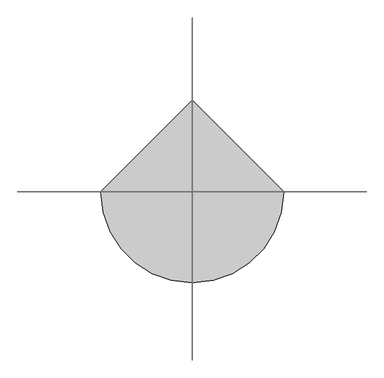
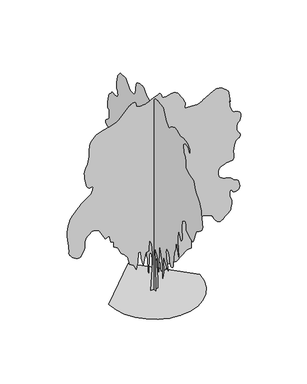
"""IFC4 building model written with IfcOpenShell, lengths in millimetres: proxy geometry, goldenchain 26164 : goldenchain 26164."""

from ifc_helpers import new_model, si_unit, origin, place, context, project, spatial, triangles, source, transform, mapped, element, save


def entourage_92130817(model_context):
    return source(origin(), model_context, "Body", "Tessellation", [
        triangles([(-0.0021439, 84.0442886, 0.0017013), (-0.0021439, -79.514705, 0.0017013), (-0.0021439, -54.9808464, 768.7285137), (-0.0021439, -30.4472354, 1202.1592524), (-0.0021439, -128.5824313, 1087.6687117), (-0.0021439, -161.2943336, 981.3544888), (-0.0021439, -161.2943336, 776.9073023), (-0.0021439, -202.1840252, 613.3465736), (-0.0021439, -226.7178838, 1406.6089096), (-0.0021439, -292.140671, 1251.2269695), (-0.0021439, -390.2761053, 932.2867716), (-0.0021439, -406.6337188, 556.102575), (-0.0021439, -447.5226474, 752.37348), (-0.0021439, -422.9887888, 1120.3813951), (-0.0021439, -398.4548939, 1226.6931473), (-0.0021439, -562.0131517, 1022.2459608), (-0.0021439, -643.7935524, 907.7528767), (-0.0021439, -570.1919403, 1161.2703238), (-0.0021439, -564.9696937, 1199.7284414), (-0.0021439, -559.9633495, 1237.6125389), (-0.0021439, -555.386267, 1274.3536102), (-0.0021439, -551.4518414, 1309.3777805), (-0.0021439, -548.3758664, 1342.1157532), (-0.0021439, -546.37181, 1371.9887844), (-0.0021439, -545.6580817, 1398.4301937), (-0.0021439, -546.8493608, 1421.534016), (-0.0021439, -550.1869114, 1442.0622688), (-0.0021439, -555.312616, 1460.4442863), (-0.0021439, -561.8709002, 1477.1091122), (-0.0021439, -569.5010668, 1492.488842), (-0.0021439, -577.8449615, 1507.0100487), (-0.0021439, -586.5470103, 1521.0994503), (-0.0021439, -614.3955648, 1489.5551548), (-0.0021439, -641.0985861, 1458.0134754), (-0.0021439, -665.5130842, 1426.4691799), (-0.0021439, -686.4960331, 1394.9248844), (-0.0021439, -702.8993196, 1363.383205), (-0.0021439, -713.5800631, 1331.8389095), (-0.0021439, -717.3950918, 1300.294614), (-0.0021439, -719.0638853, 1269.9442863), (-0.0021439, -723.7375099, 1241.7375778), (-0.0021439, -730.9130167, 1215.3215303), (-0.0021439, -740.0925436, 1190.333012), (-0.0021439, -750.773287, 1166.4189194), (-0.0021439, -762.4572395, 1143.2210621), (-0.0021439, -774.6391268, 1120.3813951), (-0.0021439, -797.2654346, 1120.6430071), (-0.0021439, -818.9620754, 1122.4794502), (-0.0021439, -838.7995274, 1127.4629396), (-0.0021439, -855.847978, 1137.1656904), (-0.0021439, -869.1753622, 1153.1626064), (-0.0021439, -877.8545563, 1177.0309896), (-0.0021439, -880.9533497, 1210.3380409), (-0.0021439, -882.6221432, 1252.4664288), (-0.0021439, -887.2956951, 1301.0338131), (-0.0021439, -894.4712019, 1354.9656956), (-0.0021439, -903.6508015, 1413.1900486), (-0.0021439, -914.3314722, 1474.6301937), (-0.0021439, -926.0154974, 1538.2190449), (-0.0021439, -938.1998554, 1602.8797783), (-0.0021439, -1003.6226789, 1758.2592476), (-0.0021439, -1028.1565012, 2036.3105896), (-0.0021439, -1134.4707968, 1611.0560234), (-0.0021439, -1093.5793247, 2028.1317284), (-0.0021439, -1118.113147, 2379.7846825), (-0.0021439, -1257.140126, 2134.4460239), (-0.0021439, -1267.5820759, 2148.5354256), (-0.0021439, -1277.5946915, 2163.0564869), (-0.0021439, -1286.7514, 2178.433746), (-0.0021439, -1294.6202511, 2195.1011879), (-0.0021439, -1300.7697304, 2213.4832054), (-0.0021439, -1304.7752998, 2234.0114582), (-0.0021439, -1306.2077705, 2257.1152805), (-0.0021439, -1304.3942184, 2284.415213), (-0.0021439, -1299.7206665, 2316.2921917), (-0.0021439, -1293.332539, 2351.3162167), (-0.0021439, -1286.3704639, 2388.0574333), (-0.0021439, -1279.9797203, 2425.0855511), (-0.0021439, -1275.3061684, 2460.9680992), (-0.0021439, -1273.4950871, 2494.2750778), (-0.0021439, -1274.6864388, 2526.5329926), (-0.0021439, -1278.0264965, 2560.0917), (-0.0021439, -1283.1522011, 2594.7116798), (-0.0021439, -1289.7079056, 2630.1702713), (-0.0021439, -1297.3381084, 2666.2889969), (-0.0021439, -1305.6820759, 2702.8396729), (-0.0021439, -1314.3840157, 2739.6188232), (-0.0021439, -1345.7607342, 2756.763707), (-0.0021439, -1376.1364964, 2771.6226837), (-0.0021439, -1404.5083111, 2781.8845573), (-0.0021439, -1429.8778381, 2785.2881287), (-0.0021439, -1451.239325, 2779.5474907), (-0.0021439, -1467.5969021, 2762.351738), (-0.0021439, -1477.9423462, 2731.439962), (-0.0021439, -1480.7337456, 2695.2194984), (-0.0021439, -1478.2292473, 2663.0124527), (-0.0021439, -1475.1534176, 2633.802317), (-0.0021439, -1476.2277706, 2606.5990356), (-0.0021439, -1486.169315, 2580.3861008), (-0.0021439, -1509.7024715, 2554.1987457), (-0.0021439, -1551.5464291, 2526.9879066), (-0.0021439, -1602.9255604, 2498.8777039), (-0.0021439, -1651.1601162, 2472.3397888), (-0.0021439, -1695.0995853, 2449.9522018), (-0.0021439, -1733.6059559, 2434.2878963), (-0.0021439, -1765.5313328, 2427.9227325), (-0.0021439, -1789.7298557, 2433.4293732), (-0.0021439, -1805.0613327, 2453.3862946), (-0.0021439, -1952.2644115, 2813.2027039), (-0.0021439, -2091.2889198, 2911.3481667), (-0.0021439, -2128.6269024, 2939.9231667), (-0.0021439, -2162.6730801, 2969.615831), (-0.0021439, -2192.1420662, 3000.6293449), (-0.0021439, -2215.746294, 3033.039576), (-0.0021439, -2232.1979061, 3067.0502907), (-0.0021439, -2240.209045, 3102.7626457), (-0.0021439, -2238.4919987, 3140.329248), (-0.0021439, -2229.7188423, 3187.039769), (-0.0021439, -2218.3701164, 3246.6282829), (-0.0021439, -2205.8758209, 3313.9381279), (-0.0021439, -2193.6685719, 3383.8138046), (-0.0021439, -2183.1783691, 3451.1236496), (-0.0021439, -2175.835358, 3510.7121635), (-0.0021439, -2173.0692478, 3557.3973953), (-0.0021439, -2164.9616032, 3599.7645767), (-0.0021439, -2142.2641514, 3649.0150589), (-0.0021439, -2107.4077034, 3703.9553101), (-0.0021439, -2062.820454, 3763.492955), (-0.0021439, -2010.9410625, 3826.4594604), (-0.0021439, -1954.194817, 3891.7374527), (-0.0021439, -1895.0179058, 3958.1331093), (-0.0021439, -1837.7740162, 4187.1141907), (-0.0021439, -1625.145425, 4236.1870674), (-0.0021439, -1453.4109947, 4317.9495186), (-0.0021439, -1454.7444889, 4324.4773178), (-0.0021439, -1458.0820759, 4341.9779938), (-0.0021439, -1462.4229446, 4367.5302132), (-0.0021439, -1466.7611973, 4398.0611984), (-0.0021439, -1470.0987843, 4430.6240364), (-0.0021439, -1471.4347492, 4462.1453682), (-0.0021439, -1469.7661011, 4489.7044418), (-0.0021439, -1464.1145565, 4515.6630318), (-0.0021439, -1454.6022011, 4544.1874535), (-0.0021439, -1441.8692574, 4574.8704643), (-0.0021439, -1426.5632149, 4607.280986), (-0.0021439, -1409.3241508, 4640.9614883), (-0.0021439, -1390.7999908, 4675.5308899), (-0.0021439, -1371.6305214, 4710.506662), (-0.0021439, -1338.9179832, 4906.7725891), (-0.0021439, -1445.2321335, 4996.7391907), (-0.0021439, -1576.0802513, 4972.2028976), (-0.0021439, -1649.6793926, 4865.8782829), (-0.0021439, -1649.6793926, 4964.0237457), (-0.0021439, -1535.1888519, 5070.3230713), (-0.0021439, -1347.0966991, 5094.8593643), (-0.0021439, -1199.8935476, 5062.1439194), (-0.0021439, -1052.6903961, 5143.9319504), (-0.0021439, -946.3761005, 5152.1111023), (-0.0021439, -938.5555023, 5148.3770279), (-0.0021439, -917.8620707, 5138.3694992), (-0.0021439, -888.4387213, 5123.7901566), (-0.0021439, -854.4407965, 5106.3400589), (-0.0021439, -820.0111393, 5087.7220093), (-0.0021439, -789.3025486, 5069.7132248), (-0.0021439, -766.462809, 5053.9653488), (-0.0021439, -750.6792521, 5038.3697891), (-0.0021439, -737.326506, 5021.3516418), (-0.0021439, -724.8322105, 5005.4770294), (-0.0021439, -711.6242231, 4993.3103302), (-0.0021439, -696.1277126, 4987.4426651), (-0.0021439, -676.7678478, 4990.465155), (-0.0021439, -651.9697975, 5004.8927628), (-0.0021439, -625.6020756, 5027.117569), (-0.0021439, -602.236605, 5051.5015457), (-0.0021439, -581.3730165, 5077.6383224), (-0.0021439, -562.5135209, 5105.2226852), (-0.0021439, -545.1577126, 5133.8994232), (-0.0021439, -528.8000991, 5163.2615845), (-0.0021439, -512.9454346, 5193.0051178), (-0.0021439, -414.8099639, 5397.4496155), (-0.0021439, -169.4723773, 5438.343631), (-0.0021439, -163.4401146, 5438.1913147), (-0.0021439, -147.2511773, 5437.2006775), (-0.0021439, -123.7660828, 5434.4828201), (-0.0021439, -95.8466569, 5429.1744232), (-0.0021439, -66.3536942, 5420.4621643), (-0.0021439, -38.1480076, 5407.4315643), (-0.0021439, -14.0911332, 5389.2710449), (-0.0021439, 3.3375856, 5370.932048), (-0.0021439, 15.1871941, 5356.7590759), (-0.0021439, 23.8896415, 5344.846431), (-0.0021439, 31.8767493, 5333.3907349), (-0.0021439, 41.5805652, 5320.4874527), (-0.0021439, 55.4332171, 5304.2826279), (-0.0021439, 75.8662495, 5282.9461395), (-0.0021439, 96.8951667, 5258.2575302), (-0.0021439, 112.9172356, 5234.5595581), (-0.0021439, 126.936765, 5213.8584961), (-0.0021439, 141.9573053, 5198.1611984), (-0.0021439, 160.9836875, 5189.5000992), (-0.0021439, 187.019453, 5189.8297302), (-0.0021439, 223.0691603, 5201.1836884), (-0.0021439, 263.6977487, 5220.8435349), (-0.0021439, 301.7494776, 5244.3891907), (-0.0021439, 337.654935, 5271.1352325), (-0.0021439, 371.8458713, 5300.4468155), (-0.0021439, 404.7490228, 5331.7146744), (-0.0021439, 436.7936874, 5364.2516418), (-0.0021439, 468.4065107, 5397.4496155), (-0.0021439, 491.2487575, 5406.0857162), (-0.0021439, 514.4465784, 5413.9090759), (-0.0021439, 538.360671, 5420.1825302), (-0.0021439, 563.3491894, 5424.0945007), (-0.0021439, 589.7652005, 5424.8560822), (-0.0021439, 617.9718727, 5421.6812759), (-0.0021439, 648.3223457, 5413.807338), (-0.0021439, 679.72181, 5404.5108124), (-0.0021439, 710.2653671, 5396.4845581), (-0.0021439, 739.0892618, 5388.0513519), (-0.0021439, 765.3401304, 5377.4595566), (-0.0021439, 788.156979, 5363.0069504), (-0.0021439, 806.6837551, 5342.991893), (-0.0021439, 820.0593922, 5315.6615845), (-0.0021439, 829.6199278, 5284.3687271), (-0.0021439, 837.4634897, 5253.4822403), (-0.0021439, 843.8769791, 5222.9771255), (-0.0021439, 849.1474422, 5192.7254837), (-0.0021439, 853.5569115, 5162.7284775), (-0.0021439, 857.3973747, 5132.8326279), (-0.0021439, 860.9483208, 5103.0379349), (-0.0021439, 866.3610718, 5073.4217194), (-0.0021439, 872.7034172, 5044.897879), (-0.0021439, 880.9050968, 5018.507048), (-0.0021439, 891.895705, 4995.3166031), (-0.0021439, 906.6073797, 4976.4444992), (-0.0021439, 925.9672445, 4962.9063721), (-0.0021439, 950.90751, 4955.8451752), (-0.0021439, 981.1385862, 4952.5180527), (-0.0021439, 1014.5192522, 4950.3588821), (-0.0021439, 1049.1851595, 4950.4606201), (-0.0021439, 1083.27959, 4954.016217), (-0.0021439, 1114.9432823, 4962.1442093), (-0.0021439, 1142.314286, 4976.0125488), (-0.0021439, 1163.533485, 4996.7391907), (-0.0021439, 1185.0142233, 5025.1618744), (-0.0021439, 1212.2201935, 5059.0452713), (-0.0021439, 1241.8544312, 5094.7832062), (-0.0021439, 1270.6326164, 5128.8195007), (-0.0021439, 1295.2629444, 5157.546817), (-0.0021439, 1312.4536102, 5177.4095581), (-0.0021439, 1318.9129543, 5184.8259659), (-0.0021439, 1572.4303288, 5168.4688248), (-0.0021439, 1670.5657631, 5045.7867783), (-0.0021439, 1675.8337555, 5036.8204651), (-0.0021439, 1681.1752899, 5026.6606201), (-0.0021439, 1686.6592575, 5014.0363907), (-0.0021439, 1692.3589096, 4997.7804062), (-0.0021439, 1698.3406666, 4976.6479752), (-0.0021439, 1704.683012, 4949.4444031), (-0.0021439, 1711.4546917, 4914.9511597), (-0.0021439, 1717.9875778, 4876.8767395), (-0.0021439, 1723.6619408, 4839.6656387), (-0.0021439, 1728.6225391, 4803.1402519), (-0.0021439, 1733.00919, 4767.2247116), (-0.0021439, 1736.9665066, 4731.7155418), (-0.0021439, 1740.6392475, 4696.5112953), (-0.0021439, 1744.1673752, 4661.4337852), (-0.0021439, 1726.808987, 4636.8466232), (-0.0021439, 1710.4538807, 4611.9798271), (-0.0021439, 1696.1003963, 4586.5546349), (-0.0021439, 1684.7516705, 4560.2402527), (-0.0021439, 1677.408514, 4532.8082062), (-0.0021439, 1675.0717381, 4503.9282829), (-0.0021439, 1678.7446243, 4473.3467194), (-0.0021439, 1687.7336105, 4446.5242287), (-0.0021439, 1700.5834076, 4427.9823372), (-0.0021439, 1717.1544891, 4416.0444031), (-0.0021439, 1737.3016605, 4408.9576263), (-0.0021439, 1760.8805992, 4405.0206573), (-0.0021439, 1787.7511974, 4402.5315651), (-0.0021439, 1817.7689873, 4399.7375496), (-0.0021439, 1846.9991798, 4399.6105225), (-0.0021439, 1872.3687069, 4403.8015457), (-0.0021439, 1895.0179058, 4408.5259666), (-0.0021439, 1916.094817, 4410.1261597), (-0.0021439, 1936.7425392, 4404.8683411), (-0.0021439, 1958.1038807, 4389.0187271), (-0.0021439, 1981.3271725, 4358.8435341), (-0.0021439, 2004.8831474, 4328.2872597), (-0.0021439, 2026.5797882, 4309.5930519), (-0.0021439, 2046.5593826, 4296.6136116), (-0.0021439, 2064.9668346, 4283.2278008), (-0.0021439, 2081.9416706, 4263.2380325), (-0.0021439, 2097.6312653, 4230.5228783), (-0.0021439, 2112.1752903, 4178.9353294), (-0.0021439, 2125.1928097, 4121.9123566), (-0.0021439, 2136.208707, 4075.3541519), (-0.0021439, 2145.220657, 4036.6698853), (-0.0021439, 2152.2311302, 4003.269017), (-0.0021439, 2157.2373653, 3972.5857155), (-0.0021439, 2160.239653, 3942.0294411), (-0.0021439, 2161.2429348, 3909.0602325), (-0.0021439, 2158.6191124, 3878.529538), (-0.0021439, 2151.2761013, 3856.1774139), (-0.0021439, 2139.9984467, 3840.6074341), (-0.0021439, 2125.5737457, 3830.4725876), (-0.0021439, 2108.7894505, 3824.4276077), (-0.0021439, 2090.4303967, 3821.0746147), (-0.0021439, 2071.2837456, 3819.093631), (-0.0021439, 2071.2837456, 3606.4699814), (-0.0021439, 2071.4514679, 3602.8379356), (-0.0021439, 2072.6198559, 3598.3167), (-0.0021439, 2075.7897205, 3592.093824), (-0.0021439, 2081.9671051, 3583.305407), (-0.0021439, 2092.1472977, 3571.0625496), (-0.0021439, 2107.334016, 3554.5525108), (-0.0021439, 2128.5303967, 3532.8863914), (-0.0021439, 2153.3512653, 3510.1278969), (-0.0021439, 2177.8850876, 3490.1125488), (-0.0021439, 2200.8441513, 3471.4944992), (-0.0021439, 2220.9432152, 3453.054055), (-0.0021439, 2236.8944218, 3433.4453682), (-0.0021439, 2247.4099136, 3411.4234566), (-0.0021439, 2251.1996532, 3385.6677612), (-0.0021439, 2244.7632729, 3361.4363914), (-0.0021439, 2226.7369022, 3344.0880318), (-0.0021439, 2199.0560337, 3332.4547302), (-0.0021439, 2163.6509274, 3325.3935333), (-0.0021439, 2122.4495178, 3321.7614876), (-0.0021439, 2077.3874428, 3320.440638), (-0.0021439, 2030.394817, 3320.2374527), (-0.0021439, 2016.5671726, 3321.7614876), (-0.0021439, 2003.8823364, 3321.9393837), (-0.0021439, 1993.4861687, 3319.3991318), (-0.0021439, 1986.5265644, 3312.7698853), (-0.0021439, 1984.1415356, 3300.704924), (-0.0021439, 1987.4789772, 3281.8325294), (-0.0021439, 1997.6847496, 3254.8324333), (-0.0021439, 2015.3987846, 3226.9687271), (-0.0021439, 2039.2646244, 3205.2770279), (-0.0021439, 2067.4229347, 3187.8780899), (-0.0021439, 2098.0122013, 3172.892086), (-0.0021439, 2129.1729446, 3158.4903488), (-0.0021439, 2159.0484467, 3142.8183403), (-0.0021439, 2185.7769024, 3123.9715256), (-0.0021439, 2209.1905895, 3107.7664101), (-0.0021439, 2229.8839485, 3098.4193062), (-0.0021439, 2247.1458309, 3091.789769), (-0.0021439, 2260.259856, 3083.7379349), (-0.0021439, 2268.5097885, 3070.0983604), (-0.0021439, 2271.1792477, 3046.7303101), (-0.0021439, 2267.5547596, 3009.4939201), (-0.0021439, 2258.1617283, 2968.2188232), (-0.0021439, 2244.4762264, 2934.6653481), (-0.0021439, 2227.2144894, 2907.5635139), (-0.0021439, 2207.0926071, 2885.592762), (-0.0021439, 2184.8218735, 2867.5078194), (-0.0021439, 2161.1236107, 2851.9884178), (-0.0021439, 2136.7091125, 2837.7389969), (-0.0021439, 2128.1010624, 2820.1877426), (-0.0021439, 2120.4252228, 2802.3315651), (-0.0021439, 2114.6061012, 2783.8911209), (-0.0021439, 2111.5783791, 2764.6123558), (-0.0021439, 2112.2691799, 2744.1653481), (-0.0021439, 2117.6108597, 2722.2960434), (-0.0021439, 2128.5303967, 2698.7248077), (-0.0021439, 2148.3677032, 2676.3473946), (-0.0021439, 2177.0748173, 2656.8148659), (-0.0021439, 2210.5012653, 2637.9933403), (-0.0021439, 2244.4991901, 2617.7495178), (-0.0021439, 2274.9232052, 2593.9245186), (-0.0021439, 2297.620657, 2564.3841705), (-0.0021439, 2308.446159, 2526.9879066), (-0.0021439, 2310.9024044, 2485.6212456), (-0.0021439, 2311.0675106, 2444.3970177), (-0.0021439, 2308.6595181, 2401.4558887), (-0.0021439, 2303.3915257, 2354.9408501), (-0.0021439, 2294.9740162, 2302.9877712), (-0.0021439, 2283.1248848, 2243.7396435), (-0.0021439, 2267.5547596, 2175.3349525), (-0.0021439, 2251.3672302, 2117.0648174), (-0.0021439, 2237.1813229, 2082.6833405), (-0.0021439, 2223.9962265, 2062.0356182), (-0.0021439, 2210.8111301, 2044.9642765), (-0.0021439, 2196.6252228, 2021.3144119), (-0.0021439, 2180.4352226, 1980.9232727), (-0.0021439, 2161.2429348, 1913.6411877), (-0.0021439, 2144.2656281, 1837.9644115), (-0.0021439, 2133.5848846, 1778.8840061), (-0.0021439, 2126.4805218, 1735.9681664), (-0.0021439, 2120.2346821, 1708.7877033), (-0.0021439, 2112.1270374, 1696.9131374), (-0.0021439, 2099.4422012, 1699.9180412), (-0.0021439, 2079.4626068, 1717.370319), (-0.0021439, 2055.4062263, 1753.7304543), (-0.0021439, 2032.2085144, 1808.9728672), (-0.0021439, 2009.7244217, 1875.9475582), (-0.0021439, 1987.8118057, 1947.4968246), (-0.0021439, 1966.3309948, 2016.4731377), (-0.0021439, 1945.1347595, 2075.7211201), (-0.0021439, 1924.0831375, 2118.0884468), (-0.0021439, 1898.5232151, 2149.1551552), (-0.0021439, 1864.8097206, 2179.3659565), (-0.0021439, 1824.3018734, 2208.8579063), (-0.0021439, 1778.3583115, 2237.7782341), (-0.0021439, 1728.3354927, 2266.2695183), (-0.0021439, 1675.5974327, 2294.4762268), (-0.0021439, 1621.4979733, 2322.5380314), (-0.0021439, 1576.1971046, 2351.8395859), (-0.0021439, 1532.4709946, 2378.2097786), (-0.0021439, 1491.8919308, 2398.715213), (-0.0021439, 1456.032201, 2410.4220566), (-0.0021439, 1426.4667091, 2410.3966221), (-0.0021439, 1404.769923, 2395.7104546), (-0.0021439, 1392.5144211, 2363.42696), (-0.0021439, 1384.3127415, 2321.608437), (-0.0021439, 1373.9674427, 2280.2191029), (-0.0021439, 1361.8312649, 2239.1854156), (-0.0021439, 1348.2650871, 2198.4387749), (-0.0021439, 1333.6245564, 2157.9054932), (-0.0021439, 1318.270261, 2117.5168247), (-0.0021439, 1302.557848, 2077.1995182), (-0.0021439, 1122.642013, 1921.8200489), (-0.0021439, 1105.2379154, 1902.4119312), (-0.0021439, 1088.5475824, 1882.2163616), (-0.0021439, 1073.2897928, 1860.4485043), (-0.0021439, 1060.1757677, 1836.3210526), (-0.0021439, 1049.9243586, 1809.0440838), (-0.0021439, 1043.2491846, 1777.8350876), (-0.0021439, 1040.8641558, 1741.9041412), (-0.0021439, 1040.1478477, 1706.9283691), (-0.0021439, 1038.1463711, 1678.3863613), (-0.0021439, 1035.070396, 1655.2139385), (-0.0021439, 1031.1359705, 1636.3290447), (-0.0021439, 1026.5588516, 1620.6648846), (-0.0021439, 1021.5525438, 1607.1469597), (-0.0021439, 1016.3302608, 1594.7010624), (-0.0021439, 869.1271093, 1496.5656281), (-0.0021439, 852.7720757, 1324.8285816), (-0.0021439, 730.1027464, 1267.5820759), (-0.0021439, 697.3900629, 1054.9560282), (-0.0021439, 566.5419814, 1022.2459608), (-0.0021439, 578.5586898, 1016.8332098), (-0.0021439, 589.0742907, 1010.4907917), (-0.0021439, 596.5850967, 1002.2891848), (-0.0021439, 599.5873844, 991.2985765), (-0.0021439, 596.5850967, 976.5869019), (-0.0021439, 586.0694959, 957.227037), (-0.0021439, 566.5419814, 932.2867716), (-0.0021439, 542.9631517, 906.6327415), (-0.0021439, 521.098825, 885.268784), (-0.0021439, 500.6670779, 867.4837503), (-0.0021439, 481.3782844, 852.5587166), (-0.0021439, 462.9480503, 839.7799181), (-0.0021439, 445.0893293, 828.4287214), (-0.0021439, 427.5175821, 817.7962309), (-0.0021439, 415.2874784, 850.3895176), (-0.0021439, 403.27077, 878.7613323), (-0.0021439, 391.6832869, 898.6927465), (-0.0021439, 380.7384244, 905.9647591), (-0.0021439, 370.6545922, 896.3558979), (-0.0021439, 361.6401352, 865.6473072), (-0.0021439, 353.9160064, 809.6174423), (-0.0021439, 346.4306348, 755.6856325), (-0.0021439, 338.0841966, 726.6457626), (-0.0021439, 329.0239938, 711.3397928), (-0.0021439, 319.3923142, 698.6092472), (-0.0021439, 309.3313731, 677.2936152), (-0.0021439, 298.9834219, 636.2370369), (-0.0021439, 288.4932192, 564.2788201), (-0.0021439, 279.4076364, 484.1215035), (-0.0021439, 272.9001666, 423.7050605), (-0.0021439, 268.5364431, 379.7401932), (-0.0021439, 265.889766, 348.9350604), (-0.0021439, 264.5308555, 328.0029442), (-0.0021439, 264.0304863, 313.6493872), (-0.0021439, 263.9593606, 302.5851461), (-0.0021439, 239.4252477, 809.6174423), (-0.0021439, 227.0988743, 842.5688467), (-0.0021439, 214.4146195, 873.4450871), (-0.0021439, 201.0151103, 900.1709993), (-0.0021439, 186.5429559, 920.6764338), (-0.0021439, 170.6400022, 932.8836828), (-0.0021439, 152.9489127, 934.7200533), (-0.0021439, 133.1120149, 924.1105265), (-0.0021439, 115.4209072, 902.0556953), (-0.0021439, 103.7379267, 871.8474375), (-0.0021439, 97.0620442, 834.8447542), (-0.0021439, 94.3917403, 792.4038855), (-0.0021439, 94.7254953, 745.8888468), (-0.0021439, 97.0620442, 696.65348), (-0.0021439, 100.3998583, 646.0591845), (-0.0021439, 84.0442886, 237.1621046), (88.2248747, 0.0002499, 0.0), (-86.1796688, 0.0002499, 0.0), (-44.6549823, 0.000202, 805.5838949), (-36.3499433, 0.0001914, 1029.8176643), (-69.5698451, 0.0001754, 1303.8836391), (-127.7051138, 0.0001648, 1445.0670273), (-144.3149375, 0.0001861, 1137.7829493), (-227.3643014, 0.0001861, 1112.8680456), (-293.8043594, 0.000202, 797.2781519), (-351.9398915, 0.0001914, 996.5995611), (-360.2456709, 0.0001808, 1179.3068682), (-426.6844571, 0.0001808, 1179.3068682), (-443.2935451, 0.0001967, 913.5491798), (-484.8200074, 0.0002073, 730.8393293), (-551.2587936, 0.000202, 872.0227175), (-659.2240059, 0.0001967, 938.4640108), (-700.7479248, 0.0001808, 1154.3919645), (-783.7983788, 0.0001754, 1254.0539772), (-875.1545031, 0.0001754, 1328.7985428), (-974.8139723, 0.0001595, 1519.8115929), (-1082.7792572, 0.0001595, 1577.9471432), (-1082.7792572, 0.0001489, 1719.1331474), (-1157.5238228, 0.0001489, 1744.0479057), (-1199.0477417, 0.0001382, 1935.0611012), (-1315.3188423, 0.0001382, 1885.2312939), (-1464.8079735, 0.0001223, 2167.6005409), (-1498.6102707, 0.0001223, 2188.6191708), (-1532.3364098, 0.0001223, 2207.6005703), (-1565.920261, 0.000117, 2222.5153576), (-1599.2856663, 0.000117, 2231.3292091), (-1632.3590836, 0.000117, 2232.0073654), (-1665.071767, 0.000117, 2222.5153576), (-1697.3475586, 0.0001223, 2200.8213329), (-1729.1864582, 0.0001223, 2173.6305508), (-1759.8645275, 0.0001223, 2148.0374908), (-1788.2186108, 0.0001276, 2122.5893349), (-1813.0851162, 0.0001276, 2095.8354446), (-1833.3035042, 0.0001276, 2066.3206764), (-1847.7078575, 0.0001329, 2032.5919212), (-1855.1424328, 0.0001329, 1993.1966515), (-1857.4665642, 0.0001382, 1950.0978287), (-1858.4826359, 0.0001382, 1906.709634), (-1859.9354542, 0.0001435, 1863.7555698), (-1863.5676453, 0.0001435, 1821.9649521), (-1871.12169, 0.0001435, 1782.0615738), (-1884.3423946, 0.0001489, 1744.7744602), (-1904.9722401, 0.0001489, 1710.8272591), (-1925.8916027, 0.0001542, 1679.5447208), (-1941.1469215, 0.0001542, 1650.7309273), (-1954.2202515, 0.0001542, 1625.8414581), (-1968.6042572, 0.0001542, 1606.3240448), (-1987.7812843, 0.0001595, 1593.6367378), (-2015.2387653, 0.0001595, 1589.2298847), (-2054.4613712, 0.0001595, 1594.5563038), (-2100.8772881, 0.0001542, 1610.4896336), (-2146.1325199, 0.0001542, 1635.5747303), (-2188.0426071, 0.0001542, 1667.7768345), (-2224.4355892, 0.0001489, 1705.0640934), (-2253.1274426, 0.0001489, 1745.4043636), (-2271.9412651, 0.0001435, 1786.7580894), (-2278.6952133, 0.0001435, 1827.0983597), (-2278.3572979, 0.0001435, 1862.6177032), (-2278.0195278, 0.0001382, 1894.6496143), (-2278.6952133, 0.0001382, 1928.8635143), (-2281.4078384, 0.0001329, 1970.9208309), (-2287.1711494, 0.0001329, 2026.4883694), (-2297.0009274, 0.0001276, 2101.2355511), (-2311.91586, 0.0001223, 2200.8213329), (-2322.6194218, 0.0001116, 2312.733688), (-2321.2629639, 0.0001063, 2418.8346245), (-2311.0445469, 0.000101, 2516.3629738), (-2295.1619408, 9.57e-05, 2602.5603287), (-2276.8079739, 9.04e-05, 2674.6710434), (-2259.1802708, 9.04e-05, 2729.9159271), (-2245.4770374, 8.51e-05, 2765.552124), (-2223.2494698, 8.51e-05, 2800.0962364), (-2182.5714294, 7.97e-05, 2849.5754837), (-2130.4174908, 7.97e-05, 2907.6399628), (-2073.7603386, 7.44e-05, 2967.8886108), (-2019.5719311, 7.44e-05, 3023.9209465), (-1974.8248077, 6.91e-05, 3069.3361977), (-1946.496159, 6.91e-05, 3097.7588814), (-1919.5238228, 6.38e-05, 3119.3488426), (-1878.1676262, 6.38e-05, 3147.4921829), (-1828.3860718, 6.38e-05, 3180.5628387), (-1776.1357727, 5.85e-05, 3216.9864876), (-1727.37029, 5.85e-05, 3255.1373566), (-1688.0485622, 5.32e-05, 3293.4405418), (-1664.1269119, 5.32e-05, 3330.2958504), (-1652.0695084, 5.32e-05, 3362.9857155), (-1643.9338131, 4.78e-05, 3390.4430511), (-1639.0672497, 4.78e-05, 3413.5317581), (-1636.8141895, 4.78e-05, 3433.1657341), (-1636.5246723, 4.78e-05, 3450.1585922), (-1637.5405987, 4.78e-05, 3465.3983597), (-1639.2120083, 4.25e-05, 3479.8003876), (-1669.3566799, 4.25e-05, 3474.8727814), (-1698.8486298, 4.25e-05, 3472.5104256), (-1727.0325199, 4.25e-05, 3475.2029938), (-1753.2554832, 4.25e-05, 3485.5407349), (-1776.8621819, 4.25e-05, 3506.0639008), (-1797.2025101, 4.25e-05, 3539.2871635), (-1813.6185139, 3.72e-05, 3587.7501938), (-1828.0965546, 3.19e-05, 3649.192955), (-1841.9954155, 3.19e-05, 3717.1379356), (-1853.7124329, 2.66e-05, 3788.029248), (-1861.6551167, 2.13e-05, 3858.1586884), (-1864.2229832, 1.59e-05, 3923.9447891), (-1859.8161301, 1.59e-05, 3981.7552139), (-1846.8366898, 1.06e-05, 4027.907048), (-1827.3218925, 1.06e-05, 4070.527993), (-1805.6277225, 5.3e-06, 4119.6770279), (-1783.6414192, 5.3e-06, 4174.7951752), (-1763.2554543, 0.0, 4235.2725883), (-1746.3543056, -5.3e-06, 4300.5505806), (-1734.827829, -1.06e-05, 4370.0448853), (-1730.5682053, -1.06e-05, 4443.1715263), (-1731.1981087, -1.59e-05, 4512.6914108), (-1731.5358788, -2.13e-05, 4573.1941132), (-1729.2601456, -2.13e-05, 4626.8643837), (-1722.0438709, -2.66e-05, 4675.9116806), (-1707.5659756, -3.19e-05, 4722.4698853), (-1683.4969505, -3.19e-05, 4768.7234573), (-1647.5177513, -3.72e-05, 4816.881855), (-1600.690377, -3.72e-05, 4863.1860054), (-1547.4697884, -4.25e-05, 4902.5054077), (-1490.6194794, -4.25e-05, 4934.9917969), (-1432.8953865, -4.25e-05, 4960.8233597), (-1377.0611492, -4.25e-05, 4980.0768356), (-1325.8750294, -4.78e-05, 4992.9801178), (-1282.0980503, -4.78e-05, 4999.6093643), (-1235.7558208, -4.78e-05, 5007.4071442), (-1178.8064627, -4.78e-05, 5022.3172806), (-1116.9168537, -4.78e-05, 5042.3067581), (-1055.7561974, -4.78e-05, 5065.3698853), (-1000.9861393, -5.32e-05, 5089.4236496), (-958.2760283, -5.32e-05, 5112.4867767), (-933.2875099, -5.32e-05, 5132.4768356), (-667.5298216, -6.91e-05, 5414.8485535), (-644.4056517, -6.91e-05, 5430.6981674), (-621.3551691, -7.44e-05, 5445.4304077), (-598.4494452, -7.44e-05, 5458.0034775), (-575.7621672, -7.44e-05, 5467.2994217), (-553.3669862, -7.44e-05, 5472.2270279), (-531.3324663, -7.44e-05, 5471.7195007), (-509.7348747, -7.44e-05, 5464.6833023), (-494.6015325, -7.44e-05, 5448.9860046), (-488.3302946, -6.91e-05, 5425.5926651), (-485.5464529, -6.91e-05, 5398.0083023), (-480.8728283, -6.91e-05, 5369.6617767), (-468.9348215, -6.91e-05, 5344.109848), (-444.3603404, -6.38e-05, 5324.7802139), (-401.7696261, -6.38e-05, 5315.1790558), (-351.2845536, -6.38e-05, 5313.8076279), (-306.0319379, -6.38e-05, 5316.3475891), (-265.1379224, -6.38e-05, 5322.1640945), (-227.7280329, -6.38e-05, 5330.5967194), (-192.9340992, -6.38e-05, 5340.9856201), (-159.8838637, -6.91e-05, 5352.6692093), (-127.7051138, -6.91e-05, 5365.0138046), (-76.3011021, -6.91e-05, 5394.9858124), (-26.1320305, -6.91e-05, 5423.3067581), (21.5672178, -7.44e-05, 5448.2750015), (65.5619775, -7.44e-05, 5468.2139008), (104.6172789, -7.44e-05, 5481.4729752), (137.4980844, -7.44e-05, 5486.4005814), (162.9699762, -7.44e-05, 5481.295079), (179.3133463, -7.44e-05, 5468.6964294), (187.9572228, -7.44e-05, 5452.7706573), (192.3880025, -7.44e-05, 5434.2287659), (196.092591, -6.91e-05, 5413.7817581), (202.5574036, -6.91e-05, 5392.1917969), (215.2690732, -6.91e-05, 5370.1448868), (237.7143056, -6.91e-05, 5348.4020279), (275.0261451, -6.38e-05, 5338.7758713), (326.72021, -6.91e-05, 5346.5736511), (387.858048, -6.91e-05, 5362.8040558), (453.4992448, -6.91e-05, 5378.4251953), (518.703586, -6.91e-05, 5384.495755), (578.5332916, -6.91e-05, 5371.9482651), (628.0480745, -6.38e-05, 5331.7908325), (667.8549471, -6.38e-05, 5276.5453674), (702.431979, -5.85e-05, 5224.3485535), (732.6477945, -5.85e-05, 5174.6917007), (759.3787937, -5.32e-05, 5127.0667007), (783.4960716, -5.32e-05, 5080.9654449), (805.8683979, -4.78e-05, 5035.8804062), (827.3694838, -4.78e-05, 4991.303476), (819.0637407, -3.72e-05, 4841.7992294), (1101.4329878, -3.72e-05, 4825.1874527), (1128.1156614, -3.72e-05, 4827.1178581), (1154.7247204, -3.72e-05, 4829.8104263), (1181.1890207, -3.72e-05, 4834.1284767), (1207.4373459, -3.72e-05, 4840.8338814), (1233.3936104, -3.72e-05, 4850.7399628), (1258.9866703, -3.72e-05, 4864.6338821), (1284.1428383, -3.72e-05, 4883.3280899), (1314.3840157, -4.25e-05, 4906.391217), (1354.2163227, -4.25e-05, 4932.4774155), (1402.0343342, -4.25e-05, 4961.1285736), (1456.2481762, -4.78e-05, 4991.8115845), (1515.2548943, -4.78e-05, 5024.0189209), (1577.4569115, -4.78e-05, 5057.2168945), (1641.2566509, -5.32e-05, 5090.9479752), (1680.2888615, -5.32e-05, 5087.2394806), (1718.5920467, -5.32e-05, 5082.6676666), (1755.4448845, -5.32e-05, 5076.3680511), (1790.1184948, -4.78e-05, 5067.4273178), (1821.883707, -4.78e-05, 5055.0065643), (1850.0193443, -4.78e-05, 5038.2174728), (1873.796236, -4.78e-05, 5016.2211411), (1895.5158405, -4.78e-05, 4994.8090759), (1917.3800583, -4.25e-05, 4978.1972992), (1938.5180122, -4.25e-05, 4963.0331085), (1958.0582439, -4.25e-05, 4945.9899628), (1975.1269695, -4.25e-05, 4923.7139969), (1988.8557827, -3.72e-05, 4892.8786697), (1998.3730797, -3.72e-05, 4850.1051178), (2031.5912556, -2.13e-05, 4609.2622604), (2026.3130894, -2.66e-05, 4631.7411209), (2021.3982731, -2.66e-05, 4650.2068542), (2017.2097206, -2.66e-05, 4660.6972023), (2014.1109272, -2.66e-05, 4659.1984566), (2012.4624813, -2.66e-05, 4641.7233604), (2012.6326744, -2.13e-05, 4604.2584961), (2014.982095, -2.13e-05, 4542.8157349), (2024.0372108, -1.59e-05, 4472.7371635), (2041.6649139, -1.06e-05, 4412.2344612), (2064.2302517, -5.3e-06, 4361.7392876), (2088.1036491, -5.3e-06, 4321.7088821), (2109.6530605, -5.3e-06, 4292.6004845), (2125.2461494, -5.3e-06, 4274.7948853), (2131.2507248, 0.0, 4268.7751945), (2142.2438038, 0.0, 4269.5626465), (2170.3794411, 0.0, 4269.054538), (2208.3929638, 0.0, 4262.8822403), (2249.0228966, 0.0, 4246.6771248), (2285.0019505, 0.0, 4216.0955612), (2309.0709755, 5.3e-06, 4166.7686302), (2313.9605026, 1.06e-05, 4094.3532829), (2302.3145565, 1.06e-05, 4025.0874527), (2283.8411201, 1.59e-05, 3981.5264488), (2261.8803967, 1.59e-05, 3953.8150589), (2239.7721531, 1.59e-05, 3932.0472015), (2220.8644409, 2.13e-05, 3906.3423752), (2208.4894695, 2.13e-05, 3866.8453674), (2205.9977612, 2.66e-05, 3803.6756767), (2214.1080219, 2.66e-05, 3738.0166031), (2229.1931477, 3.19e-05, 3693.2617767), (2248.052607, 3.19e-05, 3662.9089783), (2267.4963329, 3.72e-05, 3640.404538), (2284.3237942, 3.72e-05, 3619.1700783), (2295.3423077, 3.72e-05, 3592.7539581), (2297.3514874, 4.25e-05, 3554.5272217), (2288.6113232, 4.25e-05, 3520.3133217), (2271.1538132, 4.25e-05, 3503.5492287), (2247.4479927, 4.25e-05, 3494.176545), (2219.9678387, 4.25e-05, 3482.1877419), (2191.1768635, 4.78e-05, 3457.5500015), (2163.5518055, 4.78e-05, 3410.2805031), (2139.5564678, 5.32e-05, 3330.2958504), (2124.616246, 5.85e-05, 3235.8585915), (2119.7039005, 6.38e-05, 3152.4703674), (2120.5978867, 6.91e-05, 3080.9947884), (2123.0922112, 7.44e-05, 3022.3207535), (2122.9702709, 7.44e-05, 2977.2865837), (2116.0208405, 7.44e-05, 2946.7811783), (2098.0325489, 7.97e-05, 2931.6681473), (2075.2233307, 7.97e-05, 2926.3088814), (2054.8856186, 7.97e-05, 2923.4387077), (2034.4005318, 7.97e-05, 2921.4065643), (2011.1568924, 7.97e-05, 2918.688707), (1982.5362556, 7.97e-05, 2913.6343643), (1945.927153, 7.97e-05, 2904.642762), (1898.7111397, 7.97e-05, 2890.1392868), (1848.9295853, 7.97e-05, 2873.0196922), (1806.557317, 7.97e-05, 2855.9000977), (1771.8863228, 8.51e-05, 2836.7483597), (1745.2036491, 8.51e-05, 2813.5329163), (1726.8014294, 8.51e-05, 2784.1957535), (1716.9715061, 9.04e-05, 2746.7561783), (1716.0038326, 9.04e-05, 2699.1311783), (1719.3693249, 9.57e-05, 2651.9381287), (1723.6059849, 9.57e-05, 2615.4889), (1730.6011974, 9.57e-05, 2587.3202705), (1742.2496143, 0.000101, 2564.9937263), (1760.4309174, 0.000101, 2545.9693062), (1787.0425198, 0.000101, 2527.8387268), (1823.9665741, 0.000101, 2508.1053383), (1868.3733112, 0.000101, 2489.8733116), (1914.8146626, 0.0001063, 2476.1444984), (1961.2535431, 0.0001063, 2464.3056862), (2005.6604256, 0.0001063, 2451.7378487), (2045.9980797, 0.0001063, 2435.8296627), (2080.234798, 0.0001063, 2413.9679157), (2106.3358212, 0.0001116, 2383.5311108), (2130.3794117, 0.0001116, 2355.9518349), (2158.3448559, 0.0001116, 2339.8507828), (2188.0552517, 0.0001116, 2328.3978481), (2217.3287556, 0.0001116, 2314.7681568), (2243.9859947, 0.000117, 2292.1266609), (2265.8503578, 0.000117, 2253.6532825), (2280.7423267, 0.0001223, 2192.5154446), (2284.6387459, 0.0001276, 2127.6997787), (2276.3354736, 0.0001276, 2080.7503189), (2257.8595665, 0.0001276, 2048.6929733), (2231.2504349, 0.0001329, 2028.5482727), (2198.5377514, 0.0001329, 2017.3367477), (2161.758601, 0.0001329, 2012.084016), (2122.9474525, 0.0001329, 2009.8056667), (2101.7129929, 0.0001329, 2041.1618923), (2081.2050877, 0.0001276, 2068.4491802), (2062.1473846, 0.0001276, 2087.6032436), (2045.2716705, 0.0001276, 2094.5502033), (2031.301593, 0.0001276, 2085.2283886), (2020.9613811, 0.0001276, 2055.5688618), (2014.982095, 0.0001329, 2001.5023945), (2017.3316608, 0.0001382, 1943.077327), (2028.6854736, 0.0001382, 1899.1784077), (2044.8347786, 0.0001435, 1863.9969795), (2061.5657341, 0.0001435, 1831.721188), (2074.6671146, 0.0001435, 1796.5396145), (2079.9198463, 0.0001489, 1752.6433113), (2073.1151745, 0.0001489, 1694.2182438), (2060.9612652, 0.0001542, 1634.6526936), (2051.1314873, 0.0001595, 1588.8921146), (2040.8648174, 0.0001595, 1553.4438423), (2027.4027031, 0.0001595, 1524.8256763), (2007.9844116, 0.0001648, 1499.5475681), (1979.8489197, 0.0001648, 1474.1220852), (1940.2375294, 0.0001648, 1445.0670273), (1897.6468151, 0.0001701, 1411.1936588), (1860.8676647, 0.0001701, 1376.4489773), (1827.5758015, 0.0001701, 1345.0443535), (1795.4449139, 0.0001754, 1321.1937744), (1762.1530506, 0.0001754, 1309.1135525), (1725.3739002, 0.0001754, 1313.0099716), (1682.783186, 0.0001701, 1337.101815), (1643.0500008, 0.0001701, 1374.8030022), (1614.0660141, 0.0001701, 1414.9706085), (1592.3464096, 0.0001648, 1454.995927), (1574.4063709, 0.0001648, 1492.2577515), (1556.7559948, 0.0001595, 1524.1473747), (1535.9077034, 0.0001595, 1548.0437359), (1508.376535, 0.0001595, 1561.3381279), (1468.1125683, 0.0001595, 1573.6367958), (1415.0620274, 0.0001595, 1592.6208115), (1354.7472496, 0.0001542, 1612.7655121), (1292.689991, 0.0001542, 1628.5516125), (1234.4096821, 0.0001542, 1634.4596821), (1185.4282242, 0.0001542, 1624.9676743), (1151.2627224, 0.0001595, 1594.5563038), (1124.6054106, 0.0001595, 1573.5402901), (1095.6214966, 0.0001595, 1585.0667667), (1066.0584028, 0.0001542, 1612.8620178), (1037.6561394, 0.0001542, 1640.6597397), (1012.1621286, 0.0001542, 1652.1837456), (991.3138372, 0.0001542, 1631.1678772), (976.8586876, 0.0001595, 1561.3381279), (969.4749086, 0.0001648, 1473.9062553), (967.6105602, 0.0001701, 1406.9568535), (969.6679201, 0.0001701, 1354.5363613), (974.0494114, 0.0001754, 1310.6858402), (979.1599279, 0.0001754, 1269.4514385), (983.3966606, 0.0001808, 1224.8769791), (985.1645033, 0.0001808, 1171.0035959), (993.4677755, 0.000202, 830.4987986), (868.8934027, 0.000202, 805.5838949), (727.7100872, 0.0002127, 689.312867), (586.5241556, 0.000218, 589.6534341), (395.5085258, 0.000218, 597.9592134), (329.0697395, 0.000218, 556.4352945), (304.1548722, 0.0002233, 456.7733182), (277.6423372, 0.0002233, 451.6907796), (252.2182168, 0.0002233, 448.1296961), (228.9739052, 0.0002233, 447.6216966), (208.9983258, 0.0002233, 451.6907796), (193.3811286, 0.0002233, 461.8584002), (183.2117457, 0.0002233, 479.6561874), (179.5797908, 0.0002233, 506.6030528), (179.4588861, 0.000218, 541.3019886), (178.6112816, 0.000218, 579.775367), (176.311313, 0.0002127, 619.7016363), (171.8320261, 0.0002127, 658.7566652), (164.4472298, 0.0002127, 694.616395), (153.4302423, 0.0002073, 724.9541508), (138.0551089, 0.0002073, 747.4484173), (121.4691572, 0.0002073, 766.2139143), (107.062533, 0.0002073, 786.7218922), (94.4717499, 0.000202, 808.682761), (83.3338487, 0.000202, 831.8068583), (73.2856112, 0.000202, 855.8022686), (63.9638101, 0.000202, 880.376786), (55.0049729, 0.0001967, 905.2433641), (63.3100119, 0.0002127, 689.312867), (88.2248747, 0.0002339, 265.7602136), (-1213.063456, 0.0, 0.0051038), (-1180.9933931, -277.9547636, 0.0051038), (-1089.6600872, -533.209532, 0.0051038), (-946.3761005, -758.4542135, 0.0051038), (-758.4542135, -946.3761005, 0.0051038), (-533.209532, -1089.6600872, 0.0051038), (-277.9547636, -1180.9933931, 0.0051038), (5.3e-05, -1213.063456, 0.0051038), (277.9547636, -1180.9933931, 0.0051038), (533.209532, -1089.6600872, 0.0051038), (758.4542135, -946.3761005, 0.0051038), (946.3761005, -758.4542135, 0.0051038), (1089.6600872, -533.209532, 0.0051038), (1180.9933931, -277.9547636, 0.0051038), (1213.063456, 0.0001063, 0.0051038), (-0.0001591, 1213.063456, 0.0051038)], [[476, 477, 478], [475, 476, 478], [474, 475, 478], [473, 474, 478], [62, 63, 64], [472, 473, 478], [471, 472, 478], [470, 471, 478], [11, 12, 13], [11, 13, 14], [7, 8, 9], [6, 7, 9], [16, 17, 18], [469, 470, 478], [5, 6, 9], [10, 11, 14], [10, 14, 15], [468, 469, 478], [151, 152, 153], [151, 153, 154], [15, 16, 18], [467, 468, 478], [150, 151, 154], [150, 154, 155], [4, 5, 9], [15, 18, 19], [65, 66, 67], [65, 67, 68], [65, 68, 69], [65, 69, 70], [65, 70, 71], [65, 71, 72], [65, 72, 73], [65, 73, 74], [65, 74, 75], [65, 75, 76], [65, 76, 77], [466, 467, 478], [465, 466, 478], [464, 465, 478], [463, 464, 478], [15, 19, 20], [455, 456, 457], [65, 77, 78], [149, 150, 155], [149, 155, 156], [15, 20, 21], [62, 64, 65], [1, 2, 3], [493, 1, 3], [492, 493, 3], [491, 492, 3], [490, 491, 3], [489, 490, 3], [489, 3, 4], [488, 489, 4], [487, 488, 4], [486, 487, 4], [485, 486, 4], [484, 485, 4], [462, 463, 478], [462, 478, 479], [65, 78, 79], [15, 21, 22], [462, 479, 480], [461, 462, 480], [461, 480, 481], [391, 392, 393], [454, 455, 457], [440, 441, 442], [15, 22, 23], [65, 79, 80], [391, 393, 394], [390, 391, 394], [390, 394, 395], [389, 390, 395], [389, 395, 396], [388, 389, 396], [388, 396, 397], [387, 388, 397], [387, 397, 398], [386, 387, 398], [386, 398, 399], [385, 386, 399], [385, 399, 400], [384, 385, 400], [131, 132, 133], [45, 46, 47], [438, 439, 440], [383, 384, 400], [383, 400, 401], [382, 383, 401], [381, 382, 401], [380, 381, 401], [379, 380, 401], [379, 401, 402], [378, 379, 402], [378, 402, 403], [377, 378, 403], [376, 377, 403], [376, 403, 404], [375, 376, 404], [374, 375, 404], [373, 374, 404], [372, 373, 404], [371, 372, 404], [370, 371, 404], [369, 370, 404], [368, 369, 404], [367, 368, 404], [367, 404, 405], [366, 367, 405], [366, 405, 406], [366, 406, 407], [365, 366, 407], [365, 407, 408], [365, 408, 409], [364, 365, 409], [364, 409, 410], [363, 364, 410], [363, 410, 411], [15, 23, 24], [10, 15, 24], [9, 10, 24], [9, 24, 25], [9, 25, 26], [9, 26, 27], [9, 27, 28], [9, 28, 29], [179, 180, 181], [454, 457, 458], [453, 454, 458], [452, 453, 458], [461, 481, 482], [452, 458, 459], [451, 452, 459], [250, 251, 252], [9, 29, 30], [65, 80, 81], [460, 461, 482], [249, 250, 252], [249, 252, 253], [248, 249, 253], [247, 248, 253], [246, 247, 253], [246, 253, 254], [246, 254, 255], [246, 255, 256], [246, 256, 257], [246, 257, 258], [246, 258, 259], [246, 259, 260], [245, 246, 260], [245, 260, 261], [244, 245, 261], [244, 261, 262], [244, 262, 263], [244, 263, 264], [243, 244, 264], [243, 264, 265], [243, 265, 266], [243, 266, 267], [243, 267, 268], [243, 268, 269], [243, 269, 270], [243, 270, 271], [243, 271, 272], [242, 243, 272], [242, 272, 273], [241, 242, 273], [362, 363, 411], [450, 451, 459], [362, 411, 412], [483, 484, 4], [9, 30, 31], [241, 273, 274], [240, 241, 274], [449, 450, 459], [449, 459, 460], [448, 449, 460], [447, 448, 460], [446, 447, 460], [445, 446, 460], [444, 445, 460], [443, 444, 460], [442, 443, 460], [361, 362, 412], [9, 31, 32], [65, 81, 82], [106, 107, 108], [105, 106, 108], [105, 108, 109], [104, 105, 109], [103, 104, 109], [102, 103, 109], [101, 102, 109], [100, 101, 109], [99, 100, 109], [98, 99, 109], [97, 98, 109], [96, 97, 109], [95, 96, 109], [94, 95, 109], [93, 94, 109], [92, 93, 109], [45, 47, 48], [44, 45, 48], [44, 48, 49], [44, 49, 50], [44, 50, 51], [44, 51, 52], [44, 52, 53], [43, 44, 53], [43, 53, 54], [42, 43, 54], [41, 42, 54], [40, 41, 54], [40, 54, 55], [39, 40, 55], [38, 39, 55], [38, 55, 56], [37, 38, 56], [37, 56, 57], [36, 37, 57], [36, 57, 58], [35, 36, 58], [35, 58, 59], [34, 35, 59], [33, 34, 59], [33, 59, 60], [32, 33, 60], [32, 60, 61], [32, 61, 62], [239, 240, 274], [179, 181, 182], [179, 182, 183], [179, 183, 184], [179, 184, 185], [179, 185, 186], [179, 186, 187], [179, 187, 188], [179, 188, 189], [179, 189, 190], [179, 190, 191], [179, 191, 192], [179, 192, 193], [179, 193, 194], [179, 194, 195], [179, 195, 196], [179, 196, 197], [179, 197, 198], [178, 179, 198], [177, 178, 198], [177, 198, 199], [176, 177, 199], [175, 176, 199], [174, 175, 199], [442, 460, 482], [442, 482, 483], [442, 483, 4], [440, 442, 4], [438, 440, 4], [438, 4, 9], [360, 361, 412], [239, 274, 275], [174, 199, 200], [173, 174, 200], [436, 437, 438], [435, 436, 438], [434, 435, 438], [433, 434, 438], [433, 438, 9], [432, 433, 9], [431, 432, 9], [430, 431, 9], [429, 430, 9], [428, 429, 9], [427, 428, 9], [426, 427, 9], [426, 9, 32], [426, 32, 62], [426, 62, 65], [425, 426, 65], [424, 425, 65], [423, 424, 65], [422, 423, 65], [421, 422, 65], [420, 421, 65], [419, 420, 65], [418, 419, 65], [417, 418, 65], [416, 417, 65], [415, 416, 65], [414, 415, 65], [414, 65, 82], [414, 82, 83], [414, 83, 84], [414, 84, 85], [414, 85, 86], [414, 86, 87], [413, 414, 87], [238, 239, 275], [359, 360, 412], [148, 149, 156], [148, 156, 157], [148, 157, 158], [148, 158, 159], [148, 159, 160], [148, 160, 161], [148, 161, 162], [148, 162, 163], [148, 163, 164], [148, 164, 165], [148, 165, 166], [148, 166, 167], [148, 167, 168], [148, 168, 169], [148, 169, 170], [147, 148, 170], [146, 147, 170], [145, 146, 170], [144, 145, 170], [143, 144, 170], [142, 143, 170], [141, 142, 170], [140, 141, 170], [139, 140, 170], [138, 139, 170], [137, 138, 170], [136, 137, 170], [135, 136, 170], [134, 135, 170], [134, 170, 171], [359, 412, 413], [359, 413, 87], [92, 109, 110], [324, 325, 326], [323, 324, 326], [323, 326, 327], [322, 323, 327], [321, 322, 327], [321, 327, 328], [320, 321, 328], [320, 328, 329], [319, 320, 329], [319, 329, 330], [318, 319, 330], [317, 318, 330], [317, 330, 331], [317, 331, 332], [316, 317, 332], [316, 332, 333], [315, 316, 333], [314, 315, 333], [314, 333, 334], [313, 314, 334], [312, 313, 334], [312, 334, 335], [311, 312, 335], [359, 87, 88], [237, 238, 275], [358, 359, 88], [357, 358, 88], [356, 357, 88], [355, 356, 88], [354, 355, 88], [353, 354, 88], [352, 353, 88], [351, 352, 88], [350, 351, 88], [349, 350, 88], [348, 349, 88], [347, 348, 88], [346, 347, 88], [345, 346, 88], [344, 345, 88], [343, 344, 88], [342, 343, 88], [341, 342, 88], [340, 341, 88], [339, 340, 88], [338, 339, 88], [337, 338, 88], [336, 337, 88], [335, 336, 88], [311, 335, 88], [310, 311, 88], [309, 310, 88], [309, 88, 89], [309, 89, 90], [172, 173, 200], [91, 92, 110], [91, 110, 111], [91, 111, 112], [91, 112, 113], [91, 113, 114], [91, 114, 115], [91, 115, 116], [91, 116, 117], [91, 117, 118], [91, 118, 119], [91, 119, 120], [91, 120, 121], [91, 121, 122], [91, 122, 123], [91, 123, 124], [91, 124, 125], [91, 125, 126], [91, 126, 127], [91, 127, 128], [91, 128, 129], [91, 129, 130], [91, 130, 131], [91, 131, 133], [90, 91, 133], [309, 90, 133], [309, 133, 134], [309, 134, 171], [309, 171, 172], [309, 172, 200], [309, 200, 201], [309, 201, 202], [309, 202, 203], [309, 203, 204], [309, 204, 205], [309, 205, 206], [309, 206, 207], [309, 207, 208], [309, 208, 209], [308, 309, 209], [285, 286, 287], [284, 285, 287], [284, 287, 288], [283, 284, 288], [282, 283, 288], [282, 288, 289], [281, 282, 289], [237, 275, 276], [281, 289, 290], [236, 237, 276], [304, 305, 306], [303, 304, 306], [303, 306, 307], [302, 303, 307], [302, 307, 308], [301, 302, 308], [300, 301, 308], [299, 300, 308], [298, 299, 308], [297, 298, 308], [296, 297, 308], [295, 296, 308], [294, 295, 308], [293, 294, 308], [292, 293, 308], [291, 292, 308], [290, 291, 308], [281, 290, 308], [280, 281, 308], [279, 280, 308], [278, 279, 308], [277, 278, 308], [276, 277, 308], [236, 276, 308], [221, 222, 223], [220, 221, 223], [219, 220, 223], [219, 223, 224], [218, 219, 224], [218, 224, 225], [217, 218, 225], [217, 225, 226], [217, 226, 227], [216, 217, 227], [216, 227, 228], [215, 216, 228], [214, 215, 228], [213, 214, 228], [212, 213, 228], [211, 212, 228], [210, 211, 228], [209, 210, 228], [209, 228, 229], [209, 229, 230], [209, 230, 231], [209, 231, 232], [209, 232, 233], [209, 233, 234], [235, 236, 308], [235, 308, 209], [235, 209, 234], [711, 712, 713], [711, 713, 714], [711, 714, 715], [501, 502, 503], [506, 507, 508], [501, 503, 504], [494, 495, 496], [889, 494, 496], [888, 889, 496], [887, 888, 496], [887, 496, 497], [517, 518, 519], [859, 860, 861], [499, 500, 501], [499, 501, 504], [711, 715, 716], [505, 506, 508], [505, 508, 509], [505, 509, 510], [865, 866, 867], [513, 514, 515], [845, 846, 847], [515, 516, 517], [802, 803, 804], [865, 867, 868], [505, 510, 511], [865, 868, 869], [865, 869, 870], [865, 870, 871], [865, 871, 872], [865, 872, 873], [865, 873, 874], [865, 874, 875], [865, 875, 876], [865, 876, 877], [864, 865, 877], [864, 877, 878], [845, 847, 848], [844, 845, 848], [844, 848, 849], [499, 504, 505], [499, 505, 511], [499, 511, 512], [499, 512, 513], [499, 513, 515], [864, 878, 879], [499, 515, 517], [862, 863, 864], [862, 864, 879], [862, 879, 880], [861, 862, 880], [859, 861, 880], [859, 880, 881], [859, 881, 882], [859, 882, 883], [859, 883, 884], [859, 884, 885], [859, 885, 886], [859, 886, 887], [858, 859, 887], [857, 858, 887], [856, 857, 887], [856, 887, 497], [856, 497, 498], [855, 856, 498], [854, 855, 498], [853, 854, 498], [853, 498, 499], [852, 853, 499], [851, 852, 499], [759, 760, 761], [759, 761, 762], [758, 759, 762], [758, 762, 763], [758, 763, 764], [757, 758, 764], [757, 764, 765], [757, 765, 766], [756, 757, 766], [756, 766, 767], [756, 767, 768], [755, 756, 768], [755, 768, 769], [850, 851, 499], [850, 499, 517], [801, 802, 804], [801, 804, 805], [800, 801, 805], [799, 800, 805], [798, 799, 805], [797, 798, 805], [796, 797, 805], [796, 805, 806], [795, 796, 806], [794, 795, 806], [793, 794, 806], [792, 793, 806], [791, 792, 806], [791, 806, 807], [790, 791, 807], [789, 790, 807], [788, 789, 807], [787, 788, 807], [786, 787, 807], [785, 786, 807], [785, 807, 808], [784, 785, 808], [783, 784, 808], [782, 783, 808], [782, 808, 809], [781, 782, 809], [850, 517, 519], [696, 697, 698], [781, 809, 810], [780, 781, 810], [747, 748, 749], [747, 749, 750], [746, 747, 750], [745, 746, 750], [744, 745, 750], [744, 750, 751], [743, 744, 751], [742, 743, 751], [742, 751, 752], [755, 769, 770], [754, 755, 770], [639, 640, 641], [638, 639, 641], [637, 638, 641], [637, 641, 642], [636, 637, 642], [635, 636, 642], [634, 635, 642], [634, 642, 643], [633, 634, 643], [632, 633, 643], [631, 632, 643], [631, 643, 644], [631, 644, 645], [631, 645, 646], [680, 681, 682], [741, 742, 752], [672, 673, 674], [671, 672, 674], [671, 674, 675], [670, 671, 675], [670, 675, 676], [669, 670, 676], [669, 676, 677], [669, 677, 678], [669, 678, 679], [668, 669, 679], [668, 679, 680], [668, 680, 682], [667, 668, 682], [659, 660, 661], [659, 661, 662], [659, 662, 663], [658, 659, 663], [658, 663, 664], [657, 658, 664], [657, 664, 665], [656, 657, 665], [655, 656, 665], [655, 665, 666], [654, 655, 666], [654, 666, 667], [653, 654, 667], [653, 667, 682], [652, 653, 682], [651, 652, 682], [650, 651, 682], [649, 650, 682], [648, 649, 682], [647, 648, 682], [754, 770, 771], [828, 829, 830], [828, 830, 831], [827, 828, 831], [827, 831, 832], [826, 827, 832], [826, 832, 833], [826, 833, 834], [825, 826, 834], [825, 834, 835], [824, 825, 835], [824, 835, 836], [823, 824, 836], [822, 823, 836], [821, 822, 836], [820, 821, 836], [819, 820, 836], [818, 819, 836], [817, 818, 836], [817, 836, 837], [816, 817, 837], [815, 816, 837], [814, 815, 837], [813, 814, 837], [812, 813, 837], [811, 812, 837], [811, 837, 838], [810, 811, 838], [780, 810, 838], [780, 838, 839], [780, 839, 840], [780, 840, 841], [780, 841, 842], [779, 780, 842], [779, 842, 843], [778, 779, 843], [778, 843, 844], [778, 844, 849], [778, 849, 850], [778, 850, 519], [777, 778, 519], [776, 777, 519], [775, 776, 519], [774, 775, 519], [773, 774, 519], [772, 773, 519], [772, 519, 520], [772, 520, 521], [772, 521, 522], [771, 772, 522], [754, 771, 522], [753, 754, 522], [752, 753, 522], [741, 752, 522], [740, 741, 522], [739, 740, 522], [738, 739, 522], [738, 522, 523], [737, 738, 523], [737, 523, 524], [544, 545, 546], [543, 544, 546], [543, 546, 547], [542, 543, 547], [542, 547, 548], [541, 542, 548], [541, 548, 549], [541, 549, 550], [540, 541, 550], [540, 550, 551], [539, 540, 551], [538, 539, 551], [537, 538, 551], [537, 551, 552], [537, 552, 553], [537, 553, 554], [537, 554, 555], [536, 537, 555], [536, 555, 556], [535, 536, 556], [535, 556, 557], [534, 535, 557], [534, 557, 558], [533, 534, 558], [533, 558, 559], [532, 533, 559], [532, 559, 560], [531, 532, 560], [531, 560, 561], [530, 531, 561], [530, 561, 562], [529, 530, 562], [529, 562, 563], [528, 529, 563], [528, 563, 564], [527, 528, 564], [526, 527, 564], [526, 564, 565], [526, 565, 566], [525, 526, 566], [525, 566, 567], [525, 567, 568], [525, 568, 569], [525, 569, 570], [525, 570, 571], [525, 571, 572], [524, 525, 572], [737, 524, 572], [737, 572, 573], [737, 573, 574], [737, 574, 575], [737, 575, 576], [737, 576, 577], [737, 577, 578], [737, 578, 579], [737, 579, 580], [737, 580, 581], [737, 581, 582], [737, 582, 583], [737, 583, 584], [737, 584, 585], [737, 585, 586], [737, 586, 587], [737, 587, 588], [737, 588, 589], [736, 737, 589], [735, 736, 589], [734, 735, 589], [733, 734, 589], [732, 733, 589], [731, 732, 589], [730, 731, 589], [729, 730, 589], [728, 729, 589], [727, 728, 589], [726, 727, 589], [725, 726, 589], [724, 725, 589], [723, 724, 589], [722, 723, 589], [721, 722, 589], [720, 721, 589], [719, 720, 589], [718, 719, 589], [717, 718, 589], [716, 717, 589], [711, 716, 589], [710, 711, 589], [709, 710, 589], [708, 709, 589], [707, 708, 589], [706, 707, 589], [705, 706, 589], [704, 705, 589], [703, 704, 589], [702, 703, 589], [701, 702, 589], [700, 701, 589], [696, 698, 699], [631, 646, 647], [631, 647, 682], [630, 631, 682], [629, 630, 682], [628, 629, 682], [627, 628, 682], [626, 627, 682], [696, 699, 700], [695, 696, 700], [625, 626, 682], [592, 593, 594], [592, 594, 595], [591, 592, 595], [590, 591, 595], [590, 595, 596], [589, 590, 596], [589, 596, 597], [589, 597, 598], [589, 598, 599], [589, 599, 600], [589, 600, 601], [589, 601, 602], [589, 602, 603], [589, 603, 604], [589, 604, 605], [589, 605, 606], [589, 606, 607], [589, 607, 608], [589, 608, 609], [694, 695, 700], [624, 625, 682], [693, 694, 700], [623, 624, 682], [622, 623, 682], [621, 622, 682], [620, 621, 682], [619, 620, 682], [618, 619, 682], [617, 618, 682], [616, 617, 682], [615, 616, 682], [614, 615, 682], [613, 614, 682], [612, 613, 682], [611, 612, 682], [610, 611, 682], [609, 610, 682], [589, 609, 682], [589, 682, 683], [589, 683, 684], [589, 684, 685], [589, 685, 686], [692, 693, 700], [691, 692, 700], [690, 691, 700], [689, 690, 700], [589, 686, 687], [688, 689, 700], [688, 700, 589], [688, 589, 687], [904, 905, 890], [903, 904, 890], [903, 890, 891], [902, 903, 891], [902, 891, 892], [902, 892, 893], [901, 902, 893], [900, 901, 893], [900, 893, 894], [900, 894, 895], [900, 895, 896], [900, 896, 897], [900, 897, 898], [900, 898, 899]], closed=False),
    ])


if __name__ == "__main__":
    model = new_model("IFC4")
    model_context = context("Model", 3, world=origin())
    ifc_project = project(units=[si_unit("LENGTHUNIT", "METRE", prefix="MILLI")], contexts=[model_context])
    site = spatial("IfcSite", under=ifc_project)
    building = spatial("IfcBuilding", under=site)
    placement = place(None, origin())
    entourage_shape = entourage_92130817(model_context)
    element("IfcBuildingElementProxy", 1, Name="goldenchain 26164 : goldenchain 26164", ObjectType="goldenchain 26164 : goldenchain 26164", at=placement, inside=building, context=model_context, shape_type="MappedRepresentation", body=[
        mapped(entourage_shape, transform((0.0, 0.0, 0.0), x_axis=(1.0, 0.0, 0.0), y_axis=(0.0, 1.0, 0.0), z_axis=(0.0, 0.0, 1.0))),
    ])
    save(model, "model.ifc")

# Revit data of these elements
# Type "goldenchain 26164 : goldenchain 26164"
#   built-in parameter 1005195 = "RPC-16-FXGQ-QK7X-PJ74-6000-ST1L-LVER-AU"
#   Height = 0
